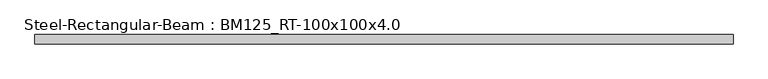
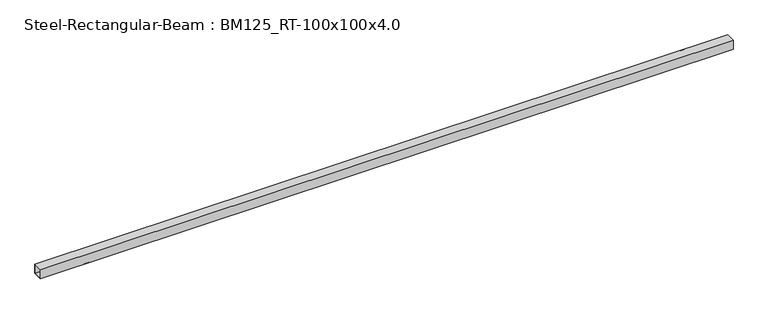
"""IFC4 building model written with IfcOpenShell, lengths in millimetres: beam geometry, Steel-Rectangular-Beam : BM125_RT-100x100x4.0."""

from ifc_helpers import new_model, si_unit, frame, origin, place, context, project, spatial, polyline, outline, extrude, source, transform, mapped, element, save


def steel_rectangular_beam_bm125_rt_100x100x4_0_bbce7aa4(model_context):
    return source(origin(), model_context, "Body", "SweptSolid", [
        extrude(outline(polyline([(-50.0, 50.0), (50.0, 50.0), (50.0, -50.0), (-50.0, -50.0), (-50.0, 50.0)]), holes=[polyline([(46.0, -46.0), (46.0, 46.0), (-46.0, 46.0), (-46.0, -46.0), (46.0, -46.0)])]), frame((-3725.0, 0.0, 0.0), z_axis=(1.0, 0.0, 0.0), x_axis=(0.0, 1.0, 0.0)), (0.0, 0.0, 1.0), 7337.3),
        extrude(outline(polyline([(-50.0, 50.0), (50.0, 50.0), (50.0, -50.0), (-50.0, -50.0), (-50.0, 50.0)]), holes=[polyline([(46.0, -46.0), (46.0, 46.0), (-46.0, 46.0), (-46.0, -46.0), (46.0, -46.0)])]), frame((-3725.0, 0.0, 0.0), z_axis=(1.0, 0.0, 0.0), x_axis=(0.0, 1.0, 0.0)), (0.0, 0.0, 1.0), 7337.3),
        extrude(outline(polyline([(-50.0, 50.0), (50.0, 50.0), (50.0, -50.0), (-50.0, -50.0), (-50.0, 50.0)]), holes=[polyline([(46.0, -46.0), (46.0, 46.0), (-46.0, 46.0), (-46.0, -46.0), (46.0, -46.0)])]), frame((-3725.0, 0.0, 0.0), z_axis=(1.0, 0.0, 0.0), x_axis=(0.0, 1.0, 0.0)), (0.0, 0.0, 1.0), 7337.3),
        extrude(outline(polyline([(-50.0, 50.0), (50.0, 50.0), (50.0, -50.0), (-50.0, -50.0), (-50.0, 50.0)]), holes=[polyline([(46.0, -46.0), (46.0, 46.0), (-46.0, 46.0), (-46.0, -46.0), (46.0, -46.0)])]), frame((-3725.0, 0.0, 0.0), z_axis=(1.0, 0.0, 0.0), x_axis=(0.0, 1.0, 0.0)), (0.0, 0.0, 1.0), 7337.3),
    ])


if __name__ == "__main__":
    model = new_model("IFC4")
    model_context = context("Model", 3, world=origin())
    ifc_project = project(units=[si_unit("LENGTHUNIT", "METRE", prefix="MILLI")], contexts=[model_context])
    site = spatial("IfcSite", under=ifc_project)
    building = spatial("IfcBuilding", under=site)
    placement = place(None, origin())
    steel_rectangular_beam_bm125_rt_100x100x4_0_shape = steel_rectangular_beam_bm125_rt_100x100x4_0_bbce7aa4(model_context)
    element("IfcBeam", 1, ObjectType="Steel-Rectangular-Beam : BM125_RT-100x100x4.0", at=placement, inside=building, context=model_context, shape_type="MappedRepresentation", body=[
        mapped(steel_rectangular_beam_bm125_rt_100x100x4_0_shape, transform((0.0, 0.0, 0.0), x_axis=(1.0, 0.0, 0.0), y_axis=(0.0, 1.0, 0.0), z_axis=(0.0, 0.0, 1.0))),
    ])
    save(model, "model.ifc")

# Revit data of these elements
# Type "Steel-Rectangular-Beam : BM125_RT-100x100x4.0"
#   t = 4 mm
#   Mass per Unit Length = 11.70 kg/m
#   Surface Area = 0.386 m²/m
#   Sectional Area = 14.95 cm²
#   Length [instance default] = 3000 mm
#   H = 100 mm
#   B = 100 mm
#   hec_material4 [instance default] = none
#   hec_material3 [instance default] = none
#   hec_material2 [instance default] = none
#   hec_material1 [instance default] = none
#   Structural Material [instance default] = none
# Element 1 (IfcBeam, "Steel-Rectangular-Beam : BM125_RT-100x100x4.0")
#   hec_material2 = S01AA010-00001_Main Steel Structure Fabrication Work_Shelter/Building_Steel Painting/Coating_for Non-Fireproofed Steel Surface, Surface Preparation, Primer, Second & Final Coat
#   hec_material1 = S03AA007-00001_Main Steel Structure Erection Work_Girth & Purlin
#   Structural Material = S01AA007-00001_Main Steel Structure Fabrication Work_Shelter/Building_Girth & Purlin
#   Materials on its faces: "S01AA010-00001_Main Steel Structure Fabrication Work_Shelter/Building_Steel Painting/Coating_for Non-Fireproofed Steel Surface, Surface Preparation, Primer, Second & Final Coat"
# Materials
#   "S01AA010-00001_Main Steel Structure Fabrication Work_Shelter/Building_Steel Painting/Coating_for Non-Fireproofed Steel Surface, Surface Preparation, Primer, Second & Final Coat": class "Metal", colour RGB 120 120 120, transparency 0, Description = "Paint finished steel", W00) Work Master Code = "S01AA010-00001", W01) Work Master_Lv1 = "Main Steel Structure Fabrication Work", W02) Work Master_Lv2 = "Shelter/Building", W03) Work Master_Spec.1 = "Steel Painting/Coating", W04) Work Master_Spec.2 = "for Non-Fireproofed Steel Surface, Surface Preparation, Primer, Second & Final Coat", Cost = 0
#   "S03AA007-00001_Main Steel Structure Erection Work_Girth & Purlin": class "Metal", colour RGB 120 120 120, transparency 0, Comments = "(30KG/M>Weight)", Description = "Structural steel 50ksi", W00) Work Master Code = "S03AA007-00001", W01) Work Master_Lv1 = "Main Steel Structure Erection Work", W02) Work Master_Lv2 = "Shelter/Building", W03) Work Master_Spec.1 = "Girth & Purlin", Cost = 0
#   "S01AA007-00001_Main Steel Structure Fabrication Work_Shelter/Building_Girth & Purlin": class "Metal", colour RGB 120 120 120, transparency 0, Comments = "(30KG/M>Weight)", Description = "Structural steel 50ksi", W00) Work Master Code = "S01AA007-00001", W01) Work Master_Lv1 = "Main Steel Structure Fabrication Work", W02) Work Master_Lv2 = "Shelter/Building", W03) Work Master_Spec.1 = "Girth & Purlin", Cost = 0
